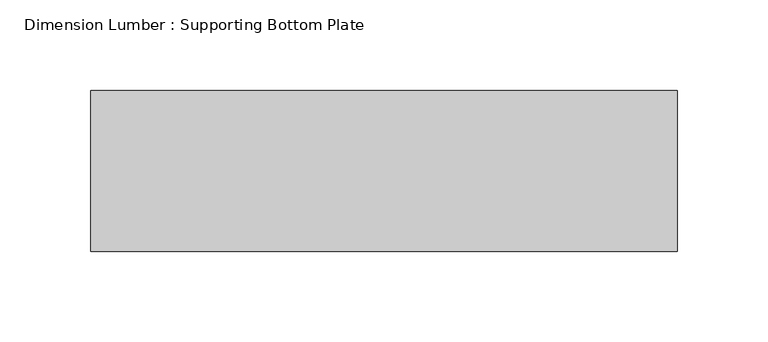
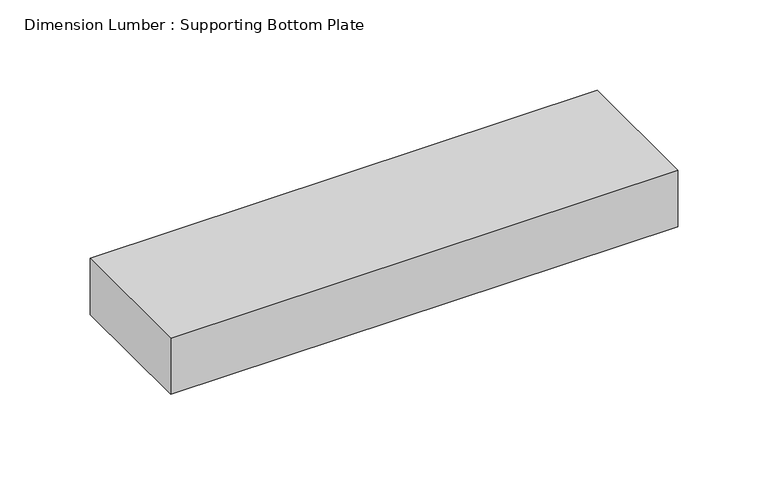
"""IFC4 building model written with IfcOpenShell, lengths in millimetres: beam geometry, Dimension Lumber : Supporting Bottom Plate."""

from ifc_helpers import new_model, si_unit, frame, origin, place, context, project, spatial, polyline, outline, extrude, source, transform, mapped, element, save


def dimension_lumber_supporting_bottom_plate_f386abe9(model_context):
    return source(origin(), model_context, "Body", "SweptSolid", [
        extrude(outline(polyline([(184.15, 44.45), (184.15, -44.45), (-139.7, -44.45), (-139.7, 44.45), (184.15, 44.45)])), frame((0.0, 0.0, -19.05), z_axis=(0.0, 0.0, 1.0), x_axis=(1.0, 0.0, 0.0)), (0.0, 0.0, 1.0), 38.1),
    ])


if __name__ == "__main__":
    model = new_model("IFC4")
    model_context = context("Model", 3, world=origin())
    ifc_project = project(units=[si_unit("LENGTHUNIT", "METRE", prefix="MILLI")], contexts=[model_context])
    site = spatial("IfcSite", under=ifc_project)
    building = spatial("IfcBuilding", under=site)
    placement = place(None, origin())
    dimension_lumber_supporting_bottom_plate_shape = dimension_lumber_supporting_bottom_plate_f386abe9(model_context)
    element("IfcBeam", 1, ObjectType="Dimension Lumber : Supporting Bottom Plate", at=placement, inside=building, context=model_context, shape_type="MappedRepresentation", body=[
        mapped(dimension_lumber_supporting_bottom_plate_shape, transform((0.0, 0.0, 0.0), x_axis=(1.0, 0.0, 0.0), y_axis=(0.0, 1.0, 0.0), z_axis=(0.0, 0.0, 1.0))),
    ])
    save(model, "model.ifc")

# Revit data of these elements
# Type "Dimension Lumber : Supporting Bottom Plate"
#   Assembly Code = "B10"
#   A = 0.0364583 SF
#   Length [instance default] = 5' - 0"
#   b = 0' - 3 1/2"
#   d = 0' - 1 1/2"
#   Structural Material [instance default] = Softwood, Lumber
# Element 1 (IfcBeam, "Dimension Lumber : Supporting Bottom Plate")
#   Structural Material = Douglas Fir #2
#   Materials on its faces: "Douglas Fir #2"
# Materials
#   "Softwood, Lumber": class "Wood", colour RGB 223 192 134, transparency 0, Description = "Pinus Echinata", Cost = 0
#   "Douglas Fir #2": class "Wood", colour RGB 223 192 134, transparency 0, Description = "Pinus Echinata", Cost = 0
